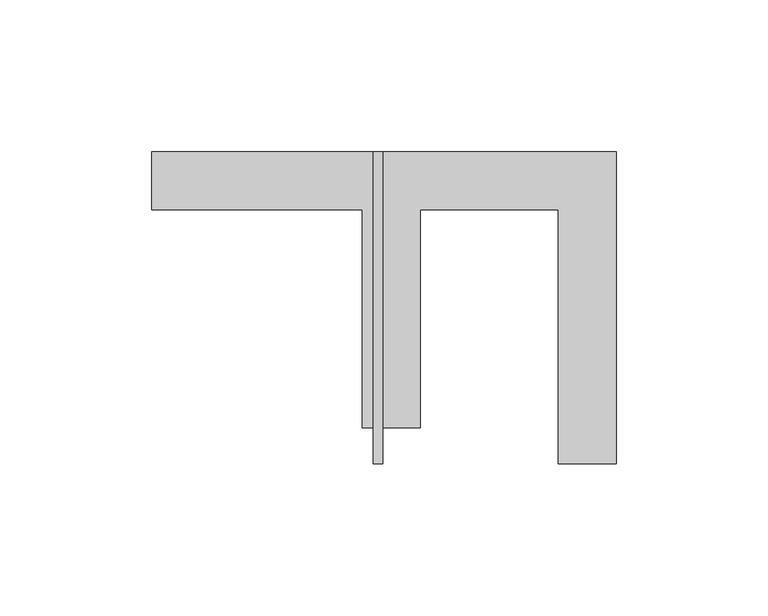
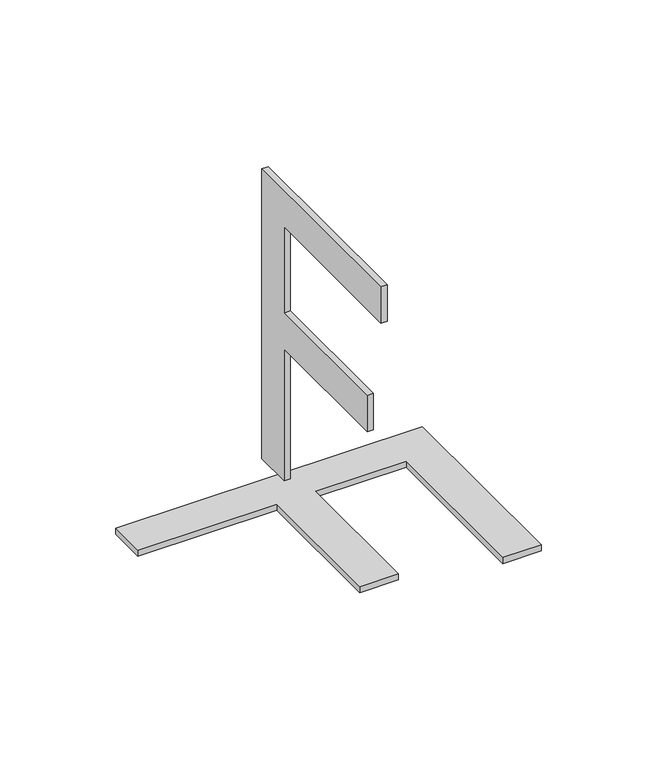
"""IFC4 building model written with IfcOpenShell, lengths in millimetres: proxy geometry, Grid Number2_FedEx : Grid Number2_FedEx."""

from ifc_helpers import new_model, si_unit, frame, origin, origin_with_axes, place, context, project, spatial, polyline, outline, extrude, source, transform, mapped, element, save


def entourage_dc536b8d(model_context):
    return source(origin(), model_context, "Body", "SweptSolid", [
        extrude(outline(polyline([(-184.2739267, 270.3629942), (-31.1785101, 270.3629942), (-31.1785101, 167.5020112), (-50.3154372, 167.5020112), (-50.3154372, 251.2260671), (-95.765639, 251.2260671), (-95.765639, 179.4625906), (-114.9025661, 179.4625906), (-114.9025661, 251.2260671), (-184.2739267, 251.2260671), (-184.2739267, 270.3629942)])), origin_with_axes(), (0.0, 0.0, 1.0), 3.175),
        extrude(outline(polyline([(270.3629942, 14.2382753), (251.2260671, 14.2382753), (251.2260671, 83.609636), (179.4625906, 83.609636), (179.4625906, 102.7465631), (251.2260671, 102.7465631), (251.2260671, 148.1967649), (167.5020112, 148.1967649), (167.5020112, 167.333692), (270.3629942, 167.333692), (270.3629942, 14.2382753)])), frame((-111.2489267, 0.0, 0.0), z_axis=(1.0, 0.0, 0.0), x_axis=(0.0, 1.0, 0.0)), (0.0, 0.0, 1.0), 3.175),
    ])


if __name__ == "__main__":
    model = new_model("IFC4")
    model_context = context("Model", 3, world=origin())
    ifc_project = project(units=[si_unit("LENGTHUNIT", "METRE", prefix="MILLI")], contexts=[model_context])
    site = spatial("IfcSite", under=ifc_project)
    building = spatial("IfcBuilding", under=site)
    placement = place(None, origin())
    entourage_shape = entourage_dc536b8d(model_context)
    element("IfcBuildingElementProxy", 1, Name="Grid Number2_FedEx : Grid Number2_FedEx", ObjectType="Grid Number2_FedEx : Grid Number2_FedEx", at=placement, inside=building, context=model_context, shape_type="MappedRepresentation", body=[
        mapped(entourage_shape, transform((0.0, 0.0, 0.0), x_axis=(1.0, 0.0, 0.0), y_axis=(0.0, 1.0, 0.0), z_axis=(0.0, 0.0, 1.0))),
    ])
    save(model, "model.ifc")

# Revit data of these elements
# Type "Grid Number2_FedEx : Grid Number2_FedEx"
#   Grid [instance default] = "S"
#   Label Width [instance default] = 1' - 0"
#   Half Box Width2 [instance default] = 0' - 6.13846"
#   Half Box Width [instance default] = 0' - 6"
#   Robust [instance default] = yes
#   Height = 0
#   Assembly Code = ""
# Element 1 (IfcBuildingElementProxy, "Grid Number2_FedEx : Grid Number2_FedEx")
#   Grid = "F"
#   Robust = no
#   Materials on its faces: "Letter"
# Materials
#   "Letter": class "Unassigned", colour RGB 178 187 30, transparency 0, Comments = "Rendering appearance not upgraded "
